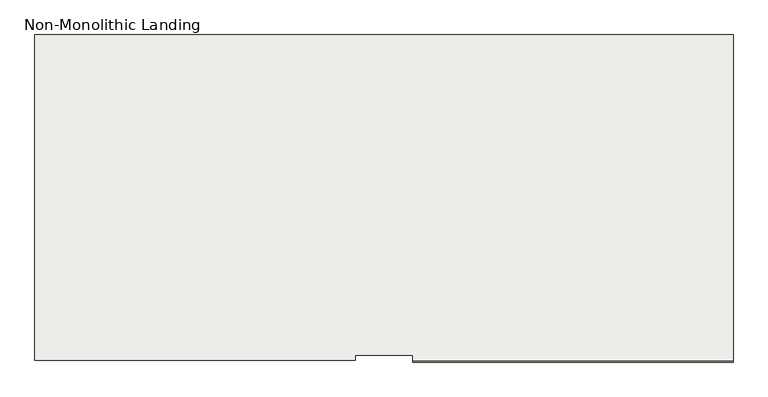
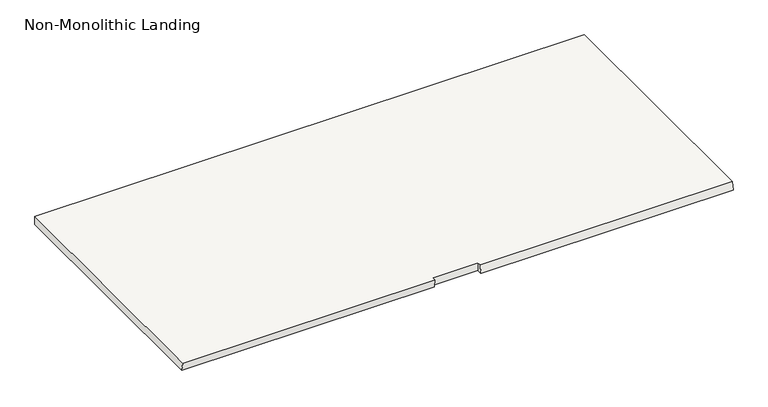
"""IFC4 building model written with IfcOpenShell, lengths in millimetres: slab geometry, Non-Monolithic Landing."""

from ifc_helpers import new_model, si_unit, origin, place, context, project, spatial, faceted_brep, source, transform, mapped, element, save


def non_monolithic_landing_f178d996(model_context):
    return source(origin(), model_context, "Body", "Brep", [
        faceted_brep([(-226.7120949, 7307.4781803, 8617.6470588), (-226.7120949, 7300.3948469, 8567.6470588), (1293.2879051, 7300.3948469, 8567.6470588), (1293.2879051, 7307.4781803, 8617.6470588), (-499.4393676, 7309.7509075, 8617.6470588), (-499.4393676, 7332.4781803, 8617.6470588), (-226.7120949, 7332.4781803, 8617.6470588), (1293.2879051, 7332.4781803, 8617.6470588), (1293.2879051, 8852.4781803, 8617.6470588), (-2019.4393676, 8852.4781803, 8617.6470588), (-2019.4393676, 7309.7509075, 8617.6470588), (-226.7120949, 7332.4781803, 8567.6470588), (-499.4393676, 7332.4781803, 8567.6470588), (-499.4393676, 7316.8342409, 8567.6470588), (-2019.4393676, 7316.8342409, 8567.6470588), (-2019.4393676, 8852.4781803, 8567.6470588), (1293.2879051, 8852.4781803, 8567.6470588), (1293.2879051, 7332.4781803, 8567.6470588)], [[[0, 1, 2, 3]], [[4, 5, 6, 0, 3, 7, 8, 9, 10]], [[11, 12, 13, 14, 15, 16, 17, 2, 1]], [[5, 4, 13, 12]], [[6, 5, 12, 11]], [[0, 6, 11, 1]], [[7, 3, 2, 17]], [[8, 7, 17, 16]], [[9, 8, 16, 15]], [[10, 9, 15, 14]], [[4, 10, 14, 13]]]),
    ])


if __name__ == "__main__":
    model = new_model("IFC4")
    model_context = context("Model", 3, world=origin())
    ifc_project = project(units=[si_unit("LENGTHUNIT", "METRE", prefix="MILLI")], contexts=[model_context])
    site = spatial("IfcSite", under=ifc_project)
    building = spatial("IfcBuilding", under=site)
    placement = place(None, origin())
    non_monolithic_landing_shape = non_monolithic_landing_f178d996(model_context)
    element("IfcSlab", 1, ObjectType="Non-Monolithic Landing", at=placement, inside=building, context=model_context, shape_type="MappedRepresentation", body=[
        mapped(non_monolithic_landing_shape, transform((0.0, 0.0, 0.0), x_axis=(1.0, 0.0, 0.0), y_axis=(0.0, 1.0, 0.0), z_axis=(0.0, 0.0, 1.0))),
    ])
    save(model, "model.ifc")
